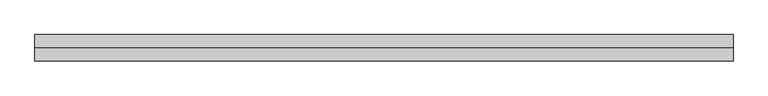
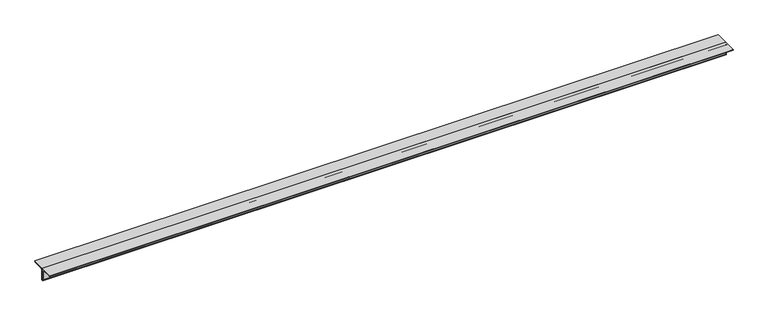
"""IFC4 building model written with IfcOpenShell, lengths in millimetres: member geometry, Steel Framing_2Ls_KS : H_SB_AR_S02_2Ls-100x100x10_VBR1."""

import ifcopenshell
import ifcopenshell.guid

model = None  # the IFC model being written
_history = None  # IfcOwnerHistory: only IFC2X3 demands one
_inside = {}  # id of a spatial element -> (the spatial element, [elements in it])
_under = {}  # id of a project, library or spatial element -> (it, [spatial elements below it])
_declared = {}  # id of a project -> (the project, [libraries it declares])
_typed = {}  # id of a type object -> (the type object, [elements of that type])
_made_of = {}  # id of a material, layer set ... -> (it, [elements and type objects made of it])


def new_model(schema):
    """Start an empty IFC model of exactly this schema.

    Asked for "IFC4X3", IfcOpenShell would pick the latest addendum, in which some entities
    have other attributes; the version numbers below select the first issue.
    IFC2X3 requires an IfcOwnerHistory on every rooted entity: one is made here for all.
    """
    global model, _history
    if schema == "IFC4X3":
        model = ifcopenshell.file(schema_version=(4, 3, 0, 0))
    else:
        model = ifcopenshell.file(schema=schema)
    _inside.clear()
    _under.clear()
    _declared.clear()
    _typed.clear()
    _made_of.clear()
    _history = None
    if model.schema == "IFC2X3":
        org = make("IfcOrganization", Name="unknown")
        user = make(
            "IfcPersonAndOrganization",
            ThePerson=make("IfcPerson", FamilyName="unknown"),
            TheOrganization=org,
        )
        app = make(
            "IfcApplication",
            ApplicationDeveloper=org,
            Version="unknown",
            ApplicationFullName="unknown",
            ApplicationIdentifier="unknown",
        )
        _history = make(
            "IfcOwnerHistory",
            OwningUser=user,
            OwningApplication=app,
            ChangeAction="ADDED",
            CreationDate=0,
        )
    return model


def make(cls, **values):
    """One entity of the class cls with the attributes given. An attribute that is None is left unset."""
    return model.create_entity(
        cls, **{name: value for name, value in values.items() if value is not None}
    )


def rooted(cls, **values):
    """An entity with a GlobalId (a new one), such as an element, a storey or a relation."""
    return make(cls, GlobalId=ifcopenshell.guid.new(), OwnerHistory=_history, **values)


def si_unit(unit_type, name, prefix=None):
    """IfcSIUnit, for example si_unit("LENGTHUNIT", "METRE", prefix="MILLI")."""
    return make("IfcSIUnit", UnitType=unit_type, Prefix=prefix, Name=name)


def assignment(units):
    """IfcUnitAssignment: the units of a project."""
    return None if units is None else make("IfcUnitAssignment", Units=units)


def point(xyz):
    """IfcCartesianPoint."""
    return None if xyz is None else make("IfcCartesianPoint", Coordinates=xyz)


def direction(xyz):
    """IfcDirection."""
    return None if xyz is None else make("IfcDirection", DirectionRatios=xyz)


def frame(location, z_axis=None, x_axis=None):
    """IfcAxis2Placement3D, a coordinate frame: its origin and axes. An axis left out is left unset."""
    return make(
        "IfcAxis2Placement3D",
        Location=point(location),
        Axis=direction(z_axis),
        RefDirection=direction(x_axis),
    )


def frame_2d(location, x_axis=None):
    """IfcAxis2Placement2D, a coordinate frame in the plane: its origin and x axis."""
    return make(
        "IfcAxis2Placement2D", Location=point(location), RefDirection=direction(x_axis)
    )


def origin():
    """The frame at (0, 0, 0) with its axes left unset."""
    return frame((0.0, 0.0, 0.0))


def place(relative_to, where):
    """IfcLocalPlacement: puts the frame where relative to a parent placement (None: the world)."""
    return make(
        "IfcLocalPlacement", PlacementRelTo=relative_to, RelativePlacement=where
    )


def context(
    kind, dimensions, precision=None, world=None, true_north=None, identifier=None
):
    """IfcGeometricRepresentationContext, for example the 3D "Model" context."""
    return make(
        "IfcGeometricRepresentationContext",
        ContextIdentifier=identifier,
        ContextType=kind,
        CoordinateSpaceDimension=dimensions,
        Precision=precision,
        WorldCoordinateSystem=world,
        TrueNorth=true_north,
    )


def project(units=None, contexts=None):
    """IfcProject with its units and contexts."""
    return rooted(
        "IfcProject",
        Name="project",
        RepresentationContexts=contexts,
        UnitsInContext=assignment(units),
    )


def spatial(cls, under=None, at=None, **own):
    """A site, building, storey or space (cls), placed at a placement, below another one or the project."""
    s = rooted(cls, ObjectPlacement=at, **own)
    if under is not None:
        _under.setdefault(under.id(), (under, []))[1].append(s)
    return s


def polyline(points):
    """IfcPolyline through the points."""
    return make("IfcPolyline", Points=[point(p) for p in points])


def circle_curve(where, radius):
    """IfcCircle in the frame where."""
    return make("IfcCircle", Position=where, Radius=radius)


def trimmed(basis, trim1, trim2, sense, master):
    """IfcTrimmedCurve: the piece of a basis curve between two trims."""
    return make(
        "IfcTrimmedCurve",
        BasisCurve=basis,
        Trim1=trim1,
        Trim2=trim2,
        SenseAgreement=sense,
        MasterRepresentation=master,
    )


def segment(curve, same_sense, transition):
    """IfcCompositeCurveSegment."""
    return make(
        "IfcCompositeCurveSegment",
        Transition=transition,
        SameSense=same_sense,
        ParentCurve=curve,
    )


def composite_curve(segments, self_intersect=None):
    """IfcCompositeCurve: segments joined end to end."""
    return make("IfcCompositeCurve", Segments=segments, SelfIntersect=self_intersect)


def outline(outer, holes=None, kind="AREA"):
    """IfcArbitraryClosedProfileDef: a profile drawn as a closed curve; with holes, ...WithVoids."""
    if holes is None:
        return make("IfcArbitraryClosedProfileDef", ProfileType=kind, OuterCurve=outer)
    return make(
        "IfcArbitraryProfileDefWithVoids",
        ProfileType=kind,
        OuterCurve=outer,
        InnerCurves=holes,
    )


def extrude(swept, where, along, depth):
    """IfcExtrudedAreaSolid: the profile swept, set in the frame where, extruded along a direction by depth."""
    return make(
        "IfcExtrudedAreaSolid",
        SweptArea=swept,
        Position=where,
        ExtrudedDirection=direction(along),
        Depth=depth,
    )


def shape(context_of_items, identifier, shape_type, items):
    """IfcShapeRepresentation: the items that make up one representation, for example the "Body"."""
    return make(
        "IfcShapeRepresentation",
        ContextOfItems=context_of_items,
        RepresentationIdentifier=identifier,
        RepresentationType=shape_type,
        Items=items,
    )


def source(mapping_origin, context_of_items, identifier, shape_type, items):
    """IfcRepresentationMap: a shape defined once, which mapped items show again and again."""
    return make(
        "IfcRepresentationMap",
        MappingOrigin=mapping_origin,
        MappedRepresentation=shape(context_of_items, identifier, shape_type, items),
    )


def transform(
    local_origin,
    x_axis=None,
    y_axis=None,
    z_axis=None,
    scale=None,
    scale2=None,
    scale3=None,
    uniform=True,
):
    """IfcCartesianTransformationOperator3D, or its non-uniform kind. x_axis, y_axis, z_axis: its Axis1, 2, 3."""
    if uniform:
        return make(
            "IfcCartesianTransformationOperator3D",
            Axis1=direction(x_axis),
            Axis2=direction(y_axis),
            LocalOrigin=point(local_origin),
            Scale=scale,
            Axis3=direction(z_axis),
        )
    return make(
        "IfcCartesianTransformationOperator3DnonUniform",
        Axis1=direction(x_axis),
        Axis2=direction(y_axis),
        LocalOrigin=point(local_origin),
        Scale=scale,
        Axis3=direction(z_axis),
        Scale2=scale2,
        Scale3=scale3,
    )


def mapped(mapping_source, mapping_target):
    """IfcMappedItem: shows the shape of a source again, moved by a transform."""
    return make(
        "IfcMappedItem", MappingSource=mapping_source, MappingTarget=mapping_target
    )


def made_of(thing, what):
    """Note that an element or type object is made of a material, layer set ...; save() writes the relation."""
    if what is not None:
        _made_of.setdefault(what.id(), (what, []))[1].append(thing)
    return thing


def element(
    cls,
    number,
    at=None,
    inside=None,
    cuts=None,
    type_object=None,
    material=None,
    context=None,
    identifier="Body",
    shape_type=None,
    held_by="IfcProductDefinitionShape",
    body=None,
    shapes=None,
    **own,
):
    """One element of the class cls, such as IfcWall. Its Tag is "e" and its number.

    at: its placement. inside: the storey or other place that contains it. cuts: it is an
    opening in that element (IfcRelVoidsElement). A single representation is given by context,
    identifier, shape_type and body (its items); several are given by shapes. held_by: the class
    of the entity that holds the representations. save() writes the other relations.
    """
    e = rooted(cls, Tag="e%d" % number, ObjectPlacement=at, **own)
    if body is not None:
        shapes = [shape(context, identifier, shape_type, body)]
    if shapes is not None:
        e.Representation = make(held_by, Representations=shapes)
    if inside is not None:
        _inside.setdefault(inside.id(), (inside, []))[1].append(e)
    if cuts is not None:
        rooted(
            "IfcRelVoidsElement", RelatingBuildingElement=cuts, RelatedOpeningElement=e
        )
    if type_object is not None:
        _typed.setdefault(type_object.id(), (type_object, []))[1].append(e)
    return made_of(e, material)


def aggregate(whole, parts):
    """IfcRelAggregates: a whole, such as a stair, and the parts it consists of."""
    return rooted("IfcRelAggregates", RelatingObject=whole, RelatedObjects=parts)


def save(model, path):
    """Write the relations noted so far, then the file.

    IfcRelAggregates (storeys below a building ...), IfcRelContainedInSpatialStructure (elements
    in a storey), IfcRelDefinesByType, IfcRelAssociatesMaterial and IfcRelDeclares: one each for
    every whole, place, type object, material and project.
    """
    for whole, parts in _under.values():
        aggregate(whole, parts)
    for where, things in _inside.values():
        rooted(
            "IfcRelContainedInSpatialStructure",
            RelatedElements=things,
            RelatingStructure=where,
        )
    for kind, things in _typed.values():
        rooted("IfcRelDefinesByType", RelatedObjects=things, RelatingType=kind)
    for what, things in _made_of.values():
        rooted("IfcRelAssociatesMaterial", RelatedObjects=things, RelatingMaterial=what)
    for by, libraries in _declared.values():
        rooted("IfcRelDeclares", RelatingContext=by, RelatedDefinitions=libraries)
    model.write(path)


def member_17757350(model_context):
    return source(origin(), model_context, "Body", "SweptSolid", [
        extrude(outline(composite_curve([segment(polyline([(0.0, 28.2), (0.0, -71.8)]), True, "CONTINUOUS"), segment(trimmed(circle_curve(frame_2d((0.0, -61.8)), 10.0), [point((0.0, -71.8))], [point((-10.0, -61.8))], False, "CARTESIAN"), True, "CONTINUOUS"), segment(polyline([(-10.0, -61.8), (-10.0, 8.2)]), True, "CONTINUOUS"), segment(trimmed(circle_curve(frame_2d((-20.0, 8.2)), 10.0), [point((-10.0, 8.2))], [point((-20.0, 18.2))], True, "CARTESIAN"), True, "CONTINUOUS"), segment(polyline([(-20.0, 18.2), (-90.0, 18.2)]), True, "CONTINUOUS"), segment(trimmed(circle_curve(frame_2d((-90.0, 28.2)), 10.0), [point((-90.0, 18.2))], [point((-100.0, 28.2))], False, "CARTESIAN"), True, "CONTINUOUS"), segment(polyline([(-100.0, 28.2), (0.0, 28.2)]), True, "CONTINUOUS")], self_intersect=False)), frame((-2838.463978, 0.0, 0.0), z_axis=(1.0, 0.0, 0.0), x_axis=(0.0, 1.0, 0.0)), (0.0, 0.0, 1.0), 5283.025664),
        extrude(outline(composite_curve([segment(polyline([(0.0, 28.2), (100.0, 28.2)]), True, "CONTINUOUS"), segment(trimmed(circle_curve(frame_2d((90.0, 28.2)), 10.0), [point((100.0, 28.2))], [point((90.0, 18.2))], False, "CARTESIAN"), True, "CONTINUOUS"), segment(polyline([(90.0, 18.2), (20.0, 18.2)]), True, "CONTINUOUS"), segment(trimmed(circle_curve(frame_2d((20.0, 8.2)), 10.0), [point((20.0, 18.2))], [point((10.0, 8.2))], True, "CARTESIAN"), True, "CONTINUOUS"), segment(polyline([(10.0, 8.2), (10.0, -61.8)]), True, "CONTINUOUS"), segment(trimmed(circle_curve(frame_2d((0.0, -61.8)), 10.0), [point((10.0, -61.8))], [point((0.0, -71.8))], False, "CARTESIAN"), True, "CONTINUOUS"), segment(polyline([(0.0, -71.8), (0.0, 28.2)]), True, "CONTINUOUS")], self_intersect=False)), frame((-2838.463978, 0.0, 0.0), z_axis=(1.0, 0.0, 0.0), x_axis=(0.0, 1.0, 0.0)), (0.0, 0.0, 1.0), 5283.025664),
    ])


if __name__ == "__main__":
    model = new_model("IFC4")
    model_context = context("Model", 3, world=origin())
    ifc_project = project(units=[si_unit("LENGTHUNIT", "METRE", prefix="MILLI")], contexts=[model_context])
    site = spatial("IfcSite", under=ifc_project)
    building = spatial("IfcBuilding", under=site)
    placement = place(None, origin())
    member_shape = member_17757350(model_context)
    element("IfcMember", 1, ObjectType="Steel Framing_2Ls_KS : H_SB_AR_S02_2Ls-100x100x10_VBR1", at=placement, inside=building, context=model_context, shape_type="MappedRepresentation", body=[
        mapped(member_shape, transform((0.0, 0.0, 0.0), x_axis=(1.0, 0.0, 0.0), y_axis=(0.0, 1.0, 0.0), z_axis=(0.0, 0.0, 1.0))),
    ])
    save(model, "model.ifc")

# Revit data of these elements
# Type "Steel Framing_2Ls_KS : H_SB_AR_S02_2Ls-100x100x10_VBR1"
#   Type Comments = "MAIN"
#   Type Mark = "VBR1"
#   H_SectionID = "2Ls-100x100x10"
#   Assembly Code = "B10"
#   Legs = "LLBB"
#   H_Ratio for Additional Steel Plate = 0.2
#   W = 0
#   Perimeter = 0.80 m²/m
#   Nominal Weight = 29.80 kgf/m
#   Length [instance default] = 1524 mm
#   Space = 0 mm
#   b = 100 mm
#   d = 100 mm
#   t = 10 mm
#   y = 28.2 mm
#   A = 0.0038 m²
#   Structural Material [instance default] = Steel, 45-345
# Element 1 (IfcMember, "Steel Framing_2Ls_KS : H_SB_AR_S02_2Ls-100x100x10_VBR1")
#   Materials on its faces: "Steel, 45-345"
# Materials
#   "Steel, 45-345": class "Metal", colour RGB 189 187 185, transparency 0, Description = "Steel 345 MPa", Cost = 0
